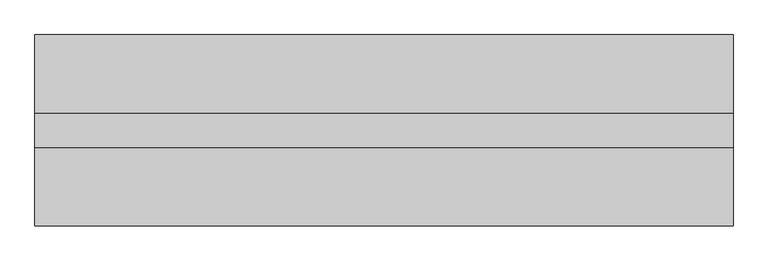
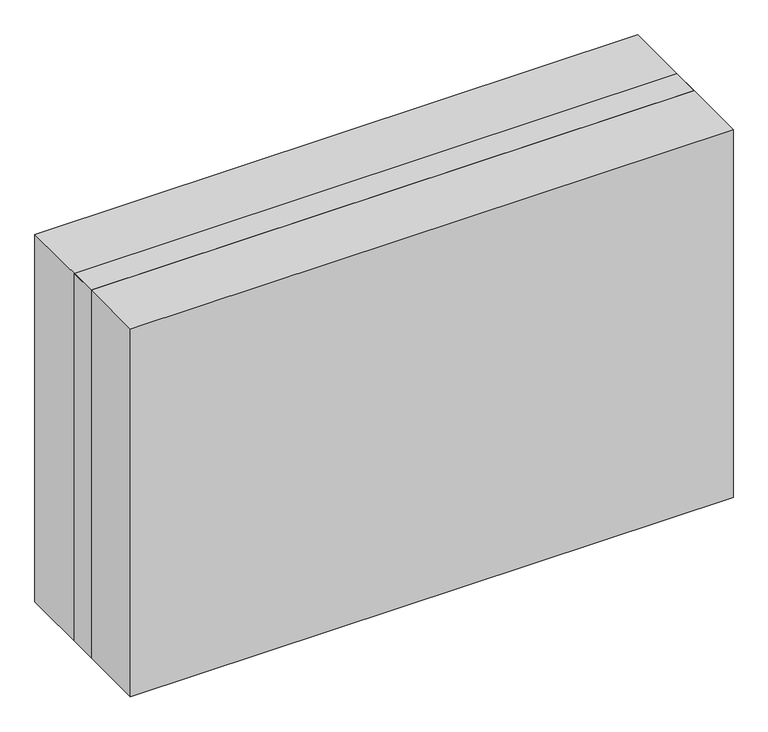
"""IFC4 building model written with IfcOpenShell, lengths in millimetres: proxy geometry, M0512 - Television, HDTV, Large Screen, 60in : M0512 - Television, HDTV, Large Screen, 60in."""

import ifcopenshell
import ifcopenshell.guid

model = None  # the IFC model being written
_history = None  # IfcOwnerHistory: only IFC2X3 demands one
_inside = {}  # id of a spatial element -> (the spatial element, [elements in it])
_under = {}  # id of a project, library or spatial element -> (it, [spatial elements below it])
_declared = {}  # id of a project -> (the project, [libraries it declares])
_typed = {}  # id of a type object -> (the type object, [elements of that type])
_made_of = {}  # id of a material, layer set ... -> (it, [elements and type objects made of it])


def new_model(schema):
    """Start an empty IFC model of exactly this schema.

    Asked for "IFC4X3", IfcOpenShell would pick the latest addendum, in which some entities
    have other attributes; the version numbers below select the first issue.
    IFC2X3 requires an IfcOwnerHistory on every rooted entity: one is made here for all.
    """
    global model, _history
    if schema == "IFC4X3":
        model = ifcopenshell.file(schema_version=(4, 3, 0, 0))
    else:
        model = ifcopenshell.file(schema=schema)
    _inside.clear()
    _under.clear()
    _declared.clear()
    _typed.clear()
    _made_of.clear()
    _history = None
    if model.schema == "IFC2X3":
        org = make("IfcOrganization", Name="unknown")
        user = make(
            "IfcPersonAndOrganization",
            ThePerson=make("IfcPerson", FamilyName="unknown"),
            TheOrganization=org,
        )
        app = make(
            "IfcApplication",
            ApplicationDeveloper=org,
            Version="unknown",
            ApplicationFullName="unknown",
            ApplicationIdentifier="unknown",
        )
        _history = make(
            "IfcOwnerHistory",
            OwningUser=user,
            OwningApplication=app,
            ChangeAction="ADDED",
            CreationDate=0,
        )
    return model


def make(cls, **values):
    """One entity of the class cls with the attributes given. An attribute that is None is left unset."""
    return model.create_entity(
        cls, **{name: value for name, value in values.items() if value is not None}
    )


def rooted(cls, **values):
    """An entity with a GlobalId (a new one), such as an element, a storey or a relation."""
    return make(cls, GlobalId=ifcopenshell.guid.new(), OwnerHistory=_history, **values)


def si_unit(unit_type, name, prefix=None):
    """IfcSIUnit, for example si_unit("LENGTHUNIT", "METRE", prefix="MILLI")."""
    return make("IfcSIUnit", UnitType=unit_type, Prefix=prefix, Name=name)


def assignment(units):
    """IfcUnitAssignment: the units of a project."""
    return None if units is None else make("IfcUnitAssignment", Units=units)


def point(xyz):
    """IfcCartesianPoint."""
    return None if xyz is None else make("IfcCartesianPoint", Coordinates=xyz)


def direction(xyz):
    """IfcDirection."""
    return None if xyz is None else make("IfcDirection", DirectionRatios=xyz)


def frame(location, z_axis=None, x_axis=None):
    """IfcAxis2Placement3D, a coordinate frame: its origin and axes. An axis left out is left unset."""
    return make(
        "IfcAxis2Placement3D",
        Location=point(location),
        Axis=direction(z_axis),
        RefDirection=direction(x_axis),
    )


def origin():
    """The frame at (0, 0, 0) with its axes left unset."""
    return frame((0.0, 0.0, 0.0))


def origin_with_axes():
    """The frame at (0, 0, 0) with the z axis (0, 0, 1) and the x axis (1, 0, 0) written out."""
    return frame((0.0, 0.0, 0.0), z_axis=(0.0, 0.0, 1.0), x_axis=(1.0, 0.0, 0.0))


def place(relative_to, where):
    """IfcLocalPlacement: puts the frame where relative to a parent placement (None: the world)."""
    return make(
        "IfcLocalPlacement", PlacementRelTo=relative_to, RelativePlacement=where
    )


def context(
    kind, dimensions, precision=None, world=None, true_north=None, identifier=None
):
    """IfcGeometricRepresentationContext, for example the 3D "Model" context."""
    return make(
        "IfcGeometricRepresentationContext",
        ContextIdentifier=identifier,
        ContextType=kind,
        CoordinateSpaceDimension=dimensions,
        Precision=precision,
        WorldCoordinateSystem=world,
        TrueNorth=true_north,
    )


def project(units=None, contexts=None):
    """IfcProject with its units and contexts."""
    return rooted(
        "IfcProject",
        Name="project",
        RepresentationContexts=contexts,
        UnitsInContext=assignment(units),
    )


def spatial(cls, under=None, at=None, **own):
    """A site, building, storey or space (cls), placed at a placement, below another one or the project."""
    s = rooted(cls, ObjectPlacement=at, **own)
    if under is not None:
        _under.setdefault(under.id(), (under, []))[1].append(s)
    return s


def polyline(points):
    """IfcPolyline through the points."""
    return make("IfcPolyline", Points=[point(p) for p in points])


def outline(outer, holes=None, kind="AREA"):
    """IfcArbitraryClosedProfileDef: a profile drawn as a closed curve; with holes, ...WithVoids."""
    if holes is None:
        return make("IfcArbitraryClosedProfileDef", ProfileType=kind, OuterCurve=outer)
    return make(
        "IfcArbitraryProfileDefWithVoids",
        ProfileType=kind,
        OuterCurve=outer,
        InnerCurves=holes,
    )


def extrude(swept, where, along, depth):
    """IfcExtrudedAreaSolid: the profile swept, set in the frame where, extruded along a direction by depth."""
    return make(
        "IfcExtrudedAreaSolid",
        SweptArea=swept,
        Position=where,
        ExtrudedDirection=direction(along),
        Depth=depth,
    )


def shape(context_of_items, identifier, shape_type, items):
    """IfcShapeRepresentation: the items that make up one representation, for example the "Body"."""
    return make(
        "IfcShapeRepresentation",
        ContextOfItems=context_of_items,
        RepresentationIdentifier=identifier,
        RepresentationType=shape_type,
        Items=items,
    )


def source(mapping_origin, context_of_items, identifier, shape_type, items):
    """IfcRepresentationMap: a shape defined once, which mapped items show again and again."""
    return make(
        "IfcRepresentationMap",
        MappingOrigin=mapping_origin,
        MappedRepresentation=shape(context_of_items, identifier, shape_type, items),
    )


def transform(
    local_origin,
    x_axis=None,
    y_axis=None,
    z_axis=None,
    scale=None,
    scale2=None,
    scale3=None,
    uniform=True,
):
    """IfcCartesianTransformationOperator3D, or its non-uniform kind. x_axis, y_axis, z_axis: its Axis1, 2, 3."""
    if uniform:
        return make(
            "IfcCartesianTransformationOperator3D",
            Axis1=direction(x_axis),
            Axis2=direction(y_axis),
            LocalOrigin=point(local_origin),
            Scale=scale,
            Axis3=direction(z_axis),
        )
    return make(
        "IfcCartesianTransformationOperator3DnonUniform",
        Axis1=direction(x_axis),
        Axis2=direction(y_axis),
        LocalOrigin=point(local_origin),
        Scale=scale,
        Axis3=direction(z_axis),
        Scale2=scale2,
        Scale3=scale3,
    )


def mapped(mapping_source, mapping_target):
    """IfcMappedItem: shows the shape of a source again, moved by a transform."""
    return make(
        "IfcMappedItem", MappingSource=mapping_source, MappingTarget=mapping_target
    )


def made_of(thing, what):
    """Note that an element or type object is made of a material, layer set ...; save() writes the relation."""
    if what is not None:
        _made_of.setdefault(what.id(), (what, []))[1].append(thing)
    return thing


def element(
    cls,
    number,
    at=None,
    inside=None,
    cuts=None,
    type_object=None,
    material=None,
    context=None,
    identifier="Body",
    shape_type=None,
    held_by="IfcProductDefinitionShape",
    body=None,
    shapes=None,
    **own,
):
    """One element of the class cls, such as IfcWall. Its Tag is "e" and its number.

    at: its placement. inside: the storey or other place that contains it. cuts: it is an
    opening in that element (IfcRelVoidsElement). A single representation is given by context,
    identifier, shape_type and body (its items); several are given by shapes. held_by: the class
    of the entity that holds the representations. save() writes the other relations.
    """
    e = rooted(cls, Tag="e%d" % number, ObjectPlacement=at, **own)
    if body is not None:
        shapes = [shape(context, identifier, shape_type, body)]
    if shapes is not None:
        e.Representation = make(held_by, Representations=shapes)
    if inside is not None:
        _inside.setdefault(inside.id(), (inside, []))[1].append(e)
    if cuts is not None:
        rooted(
            "IfcRelVoidsElement", RelatingBuildingElement=cuts, RelatedOpeningElement=e
        )
    if type_object is not None:
        _typed.setdefault(type_object.id(), (type_object, []))[1].append(e)
    return made_of(e, material)


def aggregate(whole, parts):
    """IfcRelAggregates: a whole, such as a stair, and the parts it consists of."""
    return rooted("IfcRelAggregates", RelatingObject=whole, RelatedObjects=parts)


def save(model, path):
    """Write the relations noted so far, then the file.

    IfcRelAggregates (storeys below a building ...), IfcRelContainedInSpatialStructure (elements
    in a storey), IfcRelDefinesByType, IfcRelAssociatesMaterial and IfcRelDeclares: one each for
    every whole, place, type object, material and project.
    """
    for whole, parts in _under.values():
        aggregate(whole, parts)
    for where, things in _inside.values():
        rooted(
            "IfcRelContainedInSpatialStructure",
            RelatedElements=things,
            RelatingStructure=where,
        )
    for kind, things in _typed.values():
        rooted("IfcRelDefinesByType", RelatedObjects=things, RelatingType=kind)
    for what, things in _made_of.values():
        rooted("IfcRelAssociatesMaterial", RelatedObjects=things, RelatingMaterial=what)
    for by, libraries in _declared.values():
        rooted("IfcRelDeclares", RelatingContext=by, RelatedDefinitions=libraries)
    model.write(path)


def specialty_equipment_965a27df(model_context):
    return source(origin(), model_context, "Body", "SweptSolid", [
        extrude(outline(polyline([(1016.0, 787.4), (1016.0, -787.4), (0.0, -787.4), (0.0, 787.4), (1016.0, 787.4)]), holes=[polyline([(990.6, 762.0), (25.4, 762.0), (25.4, -762.0), (990.6, -762.0), (990.6, 762.0)])]), frame((0.0, -38.1, 0.0), z_axis=(0.0, 1.0, 0.0), x_axis=(0.0, 0.0, 1.0)), (0.0, 0.0, 1.0), 76.2),
        extrude(outline(polyline([(762.0, -12.7), (-762.0, -12.7), (-762.0, 38.1), (762.0, 38.1), (762.0, -12.7)])), frame((0.0, 0.0, 25.4), z_axis=(0.0, 0.0, 1.0), x_axis=(1.0, 0.0, 0.0)), (0.0, 0.0, 1.0), 965.2),
        extrude(outline(polyline([(-787.4, 215.9), (787.4, 215.9), (787.4, -215.9), (-787.4, -215.9), (-787.4, 0.0), (-787.4, 215.9)])), origin_with_axes(), (0.0, 0.0, 1.0), 1016.0),
    ])


if __name__ == "__main__":
    model = new_model("IFC4")
    model_context = context("Model", 3, world=origin())
    ifc_project = project(units=[si_unit("LENGTHUNIT", "METRE", prefix="MILLI")], contexts=[model_context])
    site = spatial("IfcSite", under=ifc_project)
    building = spatial("IfcBuilding", under=site)
    placement = place(None, origin())
    specialty_equipment_shape = specialty_equipment_965a27df(model_context)
    element("IfcBuildingElementProxy", 1, Name="M0512 - Television, HDTV, Large Screen, 60in : M0512 - Television, HDTV, Large Screen, 60in", ObjectType="M0512 - Television, HDTV, Large Screen, 60in : M0512 - Television, HDTV, Large Screen, 60in", at=placement, inside=building, context=model_context, shape_type="MappedRepresentation", body=[
        mapped(specialty_equipment_shape, transform((0.0, 0.0, 0.0), x_axis=(1.0, 0.0, 0.0), y_axis=(0.0, 1.0, 0.0), z_axis=(0.0, 0.0, 1.0))),
    ])
    save(model, "model.ifc")

# Revit data of these elements
# Project information
#   Room Abbreviation = "BRUN1/TLTS2"
#   Room Description 2-1 = "Bedroom, Acuity Adaptable (BRUN1)"
#   Room Description 2-2 = "Toilet/Shower (TLTS2)"
#   Sheets - Total = "8"
#   Project Issue Date = "Issue Date"
#   Project Status = "Project Status"
#   Client Name = "Owner"
#   Project Address = "Enter address here"
#   Project Name = "Project Name"
#   Project Number = "Project Number"
#   Publication Date = "30-Jan-15"
# Type "M0512 - Television, HDTV, Large Screen, 60in : M0512 - Television, HDTV, Large Screen, 60in"
#   Watts2 = "0"
#   Watts1 = "240"
#   Unit_Issue = "EA"
#   UTIL_6_Misc = "-"
#   UTIL_5_NonMedGas = "-"
#   UTIL_4_MiscGas = "-"
#   UTIL_3_MedGas = "-"
#   UTIL_2_Elec = "A"
#   UTIL_1_WaterDrain = "-"
#   Nomenclature = "Television, HDTV, Large Screen, 60\""
#   NSN = ""
#   Location [instance default] = ""
#   JSN = "M0512"
#   Fund_Source_VA = "-"
#   Fund_Source_Navy = "-"
#   Fund_Source_Army = "-"
#   Fund_Source_AF = "-"
#   ELEC_Volts2 = "0"
#   ELEC_Volts1 = "120"
#   ELEC_Phase2 = "0"
#   ELEC_Phase1 = "1"
#   ELEC_HertzSwitch = "0"
#   ELEC_HertzDependent = "-1"
#   ELEC_Hertz = "60"
#   ELEC_Amps2 = "0"
#   ELEC_Amps1 = "2"
#   DetailDescription = "A high definition (HDTV) multimedia, slim design, 60\"W to 65\"W color television. The TV will have a 16.9 wide screen aspect ratio with full HD 1080p resolution and HDMI connections. TV may be LED, Plasma or LCD. TV will include a stand."
#   CAT_VA = "C"
#   CAT_Navy = "C"
#   CAT_IHS = "-"
#   CAT_Army = "C"
#   CAT_AF = "C"
#   BTUperhour = "0"
#   Weight_IP = 88
#   DIM_Width_IP = 5' - 2"
#   DIM_Height_IP = 3' - 4"
#   DIM_Depth_IP = 1' - 5"
# Element 1 (IfcBuildingElementProxy, "M0512 - Television, HDTV, Large Screen, 60in : M0512 - Television, HDTV, Large Screen, 60in")
#   Materials on its faces: "EquipSpace"
# Materials
#   "EquipSpace": class "Unassigned", colour RGB 221 217 195, transparency 0.5
